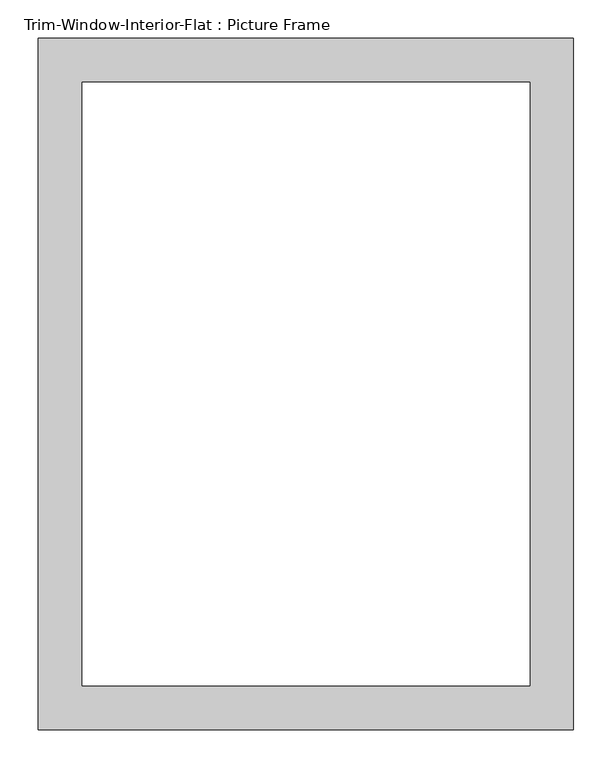
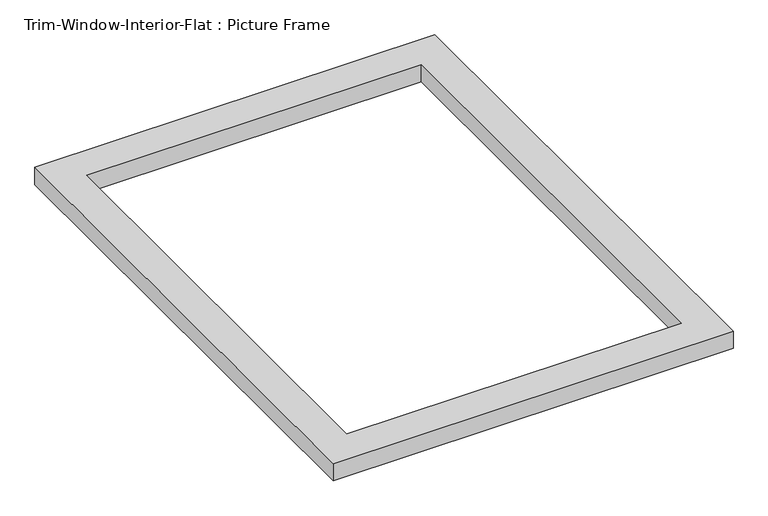
"""IFC4 building model written with IfcOpenShell, lengths in millimetres: proxy geometry, Trim-Window-Interior-Flat : Picture Frame."""

import ifcopenshell
import ifcopenshell.guid

model = None  # the IFC model being written
_history = None  # IfcOwnerHistory: only IFC2X3 demands one
_inside = {}  # id of a spatial element -> (the spatial element, [elements in it])
_under = {}  # id of a project, library or spatial element -> (it, [spatial elements below it])
_declared = {}  # id of a project -> (the project, [libraries it declares])
_typed = {}  # id of a type object -> (the type object, [elements of that type])
_made_of = {}  # id of a material, layer set ... -> (it, [elements and type objects made of it])


def new_model(schema):
    """Start an empty IFC model of exactly this schema.

    Asked for "IFC4X3", IfcOpenShell would pick the latest addendum, in which some entities
    have other attributes; the version numbers below select the first issue.
    IFC2X3 requires an IfcOwnerHistory on every rooted entity: one is made here for all.
    """
    global model, _history
    if schema == "IFC4X3":
        model = ifcopenshell.file(schema_version=(4, 3, 0, 0))
    else:
        model = ifcopenshell.file(schema=schema)
    _inside.clear()
    _under.clear()
    _declared.clear()
    _typed.clear()
    _made_of.clear()
    _history = None
    if model.schema == "IFC2X3":
        org = make("IfcOrganization", Name="unknown")
        user = make(
            "IfcPersonAndOrganization",
            ThePerson=make("IfcPerson", FamilyName="unknown"),
            TheOrganization=org,
        )
        app = make(
            "IfcApplication",
            ApplicationDeveloper=org,
            Version="unknown",
            ApplicationFullName="unknown",
            ApplicationIdentifier="unknown",
        )
        _history = make(
            "IfcOwnerHistory",
            OwningUser=user,
            OwningApplication=app,
            ChangeAction="ADDED",
            CreationDate=0,
        )
    return model


def make(cls, **values):
    """One entity of the class cls with the attributes given. An attribute that is None is left unset."""
    return model.create_entity(
        cls, **{name: value for name, value in values.items() if value is not None}
    )


def rooted(cls, **values):
    """An entity with a GlobalId (a new one), such as an element, a storey or a relation."""
    return make(cls, GlobalId=ifcopenshell.guid.new(), OwnerHistory=_history, **values)


def si_unit(unit_type, name, prefix=None):
    """IfcSIUnit, for example si_unit("LENGTHUNIT", "METRE", prefix="MILLI")."""
    return make("IfcSIUnit", UnitType=unit_type, Prefix=prefix, Name=name)


def assignment(units):
    """IfcUnitAssignment: the units of a project."""
    return None if units is None else make("IfcUnitAssignment", Units=units)


def point(xyz):
    """IfcCartesianPoint."""
    return None if xyz is None else make("IfcCartesianPoint", Coordinates=xyz)


def direction(xyz):
    """IfcDirection."""
    return None if xyz is None else make("IfcDirection", DirectionRatios=xyz)


def frame(location, z_axis=None, x_axis=None):
    """IfcAxis2Placement3D, a coordinate frame: its origin and axes. An axis left out is left unset."""
    return make(
        "IfcAxis2Placement3D",
        Location=point(location),
        Axis=direction(z_axis),
        RefDirection=direction(x_axis),
    )


def origin():
    """The frame at (0, 0, 0) with its axes left unset."""
    return frame((0.0, 0.0, 0.0))


def origin_with_axes():
    """The frame at (0, 0, 0) with the z axis (0, 0, 1) and the x axis (1, 0, 0) written out."""
    return frame((0.0, 0.0, 0.0), z_axis=(0.0, 0.0, 1.0), x_axis=(1.0, 0.0, 0.0))


def place(relative_to, where):
    """IfcLocalPlacement: puts the frame where relative to a parent placement (None: the world)."""
    return make(
        "IfcLocalPlacement", PlacementRelTo=relative_to, RelativePlacement=where
    )


def context(
    kind, dimensions, precision=None, world=None, true_north=None, identifier=None
):
    """IfcGeometricRepresentationContext, for example the 3D "Model" context."""
    return make(
        "IfcGeometricRepresentationContext",
        ContextIdentifier=identifier,
        ContextType=kind,
        CoordinateSpaceDimension=dimensions,
        Precision=precision,
        WorldCoordinateSystem=world,
        TrueNorth=true_north,
    )


def project(units=None, contexts=None):
    """IfcProject with its units and contexts."""
    return rooted(
        "IfcProject",
        Name="project",
        RepresentationContexts=contexts,
        UnitsInContext=assignment(units),
    )


def spatial(cls, under=None, at=None, **own):
    """A site, building, storey or space (cls), placed at a placement, below another one or the project."""
    s = rooted(cls, ObjectPlacement=at, **own)
    if under is not None:
        _under.setdefault(under.id(), (under, []))[1].append(s)
    return s


def polyline(points):
    """IfcPolyline through the points."""
    return make("IfcPolyline", Points=[point(p) for p in points])


def outline(outer, holes=None, kind="AREA"):
    """IfcArbitraryClosedProfileDef: a profile drawn as a closed curve; with holes, ...WithVoids."""
    if holes is None:
        return make("IfcArbitraryClosedProfileDef", ProfileType=kind, OuterCurve=outer)
    return make(
        "IfcArbitraryProfileDefWithVoids",
        ProfileType=kind,
        OuterCurve=outer,
        InnerCurves=holes,
    )


def extrude(swept, where, along, depth):
    """IfcExtrudedAreaSolid: the profile swept, set in the frame where, extruded along a direction by depth."""
    return make(
        "IfcExtrudedAreaSolid",
        SweptArea=swept,
        Position=where,
        ExtrudedDirection=direction(along),
        Depth=depth,
    )


def shape(context_of_items, identifier, shape_type, items):
    """IfcShapeRepresentation: the items that make up one representation, for example the "Body"."""
    return make(
        "IfcShapeRepresentation",
        ContextOfItems=context_of_items,
        RepresentationIdentifier=identifier,
        RepresentationType=shape_type,
        Items=items,
    )


def source(mapping_origin, context_of_items, identifier, shape_type, items):
    """IfcRepresentationMap: a shape defined once, which mapped items show again and again."""
    return make(
        "IfcRepresentationMap",
        MappingOrigin=mapping_origin,
        MappedRepresentation=shape(context_of_items, identifier, shape_type, items),
    )


def transform(
    local_origin,
    x_axis=None,
    y_axis=None,
    z_axis=None,
    scale=None,
    scale2=None,
    scale3=None,
    uniform=True,
):
    """IfcCartesianTransformationOperator3D, or its non-uniform kind. x_axis, y_axis, z_axis: its Axis1, 2, 3."""
    if uniform:
        return make(
            "IfcCartesianTransformationOperator3D",
            Axis1=direction(x_axis),
            Axis2=direction(y_axis),
            LocalOrigin=point(local_origin),
            Scale=scale,
            Axis3=direction(z_axis),
        )
    return make(
        "IfcCartesianTransformationOperator3DnonUniform",
        Axis1=direction(x_axis),
        Axis2=direction(y_axis),
        LocalOrigin=point(local_origin),
        Scale=scale,
        Axis3=direction(z_axis),
        Scale2=scale2,
        Scale3=scale3,
    )


def mapped(mapping_source, mapping_target):
    """IfcMappedItem: shows the shape of a source again, moved by a transform."""
    return make(
        "IfcMappedItem", MappingSource=mapping_source, MappingTarget=mapping_target
    )


def made_of(thing, what):
    """Note that an element or type object is made of a material, layer set ...; save() writes the relation."""
    if what is not None:
        _made_of.setdefault(what.id(), (what, []))[1].append(thing)
    return thing


def element(
    cls,
    number,
    at=None,
    inside=None,
    cuts=None,
    type_object=None,
    material=None,
    context=None,
    identifier="Body",
    shape_type=None,
    held_by="IfcProductDefinitionShape",
    body=None,
    shapes=None,
    **own,
):
    """One element of the class cls, such as IfcWall. Its Tag is "e" and its number.

    at: its placement. inside: the storey or other place that contains it. cuts: it is an
    opening in that element (IfcRelVoidsElement). A single representation is given by context,
    identifier, shape_type and body (its items); several are given by shapes. held_by: the class
    of the entity that holds the representations. save() writes the other relations.
    """
    e = rooted(cls, Tag="e%d" % number, ObjectPlacement=at, **own)
    if body is not None:
        shapes = [shape(context, identifier, shape_type, body)]
    if shapes is not None:
        e.Representation = make(held_by, Representations=shapes)
    if inside is not None:
        _inside.setdefault(inside.id(), (inside, []))[1].append(e)
    if cuts is not None:
        rooted(
            "IfcRelVoidsElement", RelatingBuildingElement=cuts, RelatedOpeningElement=e
        )
    if type_object is not None:
        _typed.setdefault(type_object.id(), (type_object, []))[1].append(e)
    return made_of(e, material)


def aggregate(whole, parts):
    """IfcRelAggregates: a whole, such as a stair, and the parts it consists of."""
    return rooted("IfcRelAggregates", RelatingObject=whole, RelatedObjects=parts)


def save(model, path):
    """Write the relations noted so far, then the file.

    IfcRelAggregates (storeys below a building ...), IfcRelContainedInSpatialStructure (elements
    in a storey), IfcRelDefinesByType, IfcRelAssociatesMaterial and IfcRelDeclares: one each for
    every whole, place, type object, material and project.
    """
    for whole, parts in _under.values():
        aggregate(whole, parts)
    for where, things in _inside.values():
        rooted(
            "IfcRelContainedInSpatialStructure",
            RelatedElements=things,
            RelatingStructure=where,
        )
    for kind, things in _typed.values():
        rooted("IfcRelDefinesByType", RelatedObjects=things, RelatingType=kind)
    for what, things in _made_of.values():
        rooted("IfcRelAssociatesMaterial", RelatedObjects=things, RelatingMaterial=what)
    for by, libraries in _declared.values():
        rooted("IfcRelDeclares", RelatingContext=by, RelatedDefinitions=libraries)
    model.write(path)


def trim_window_interior_flat_picture_frame_6a74a1f9(model_context):
    return source(origin(), model_context, "Body", "SweptSolid", [
        extrude(outline(polyline([(349.25, 44.45), (349.25, -857.25), (-349.25, -857.25), (-349.25, 44.45), (349.25, 44.45)]), holes=[polyline([(292.1, -12.7), (-292.1, -12.7), (-292.1, -800.1), (292.1, -800.1), (292.1, -12.7)])]), origin_with_axes(), (0.0, 0.0, 1.0), 31.75),
    ])


if __name__ == "__main__":
    model = new_model("IFC4")
    model_context = context("Model", 3, world=origin())
    ifc_project = project(units=[si_unit("LENGTHUNIT", "METRE", prefix="MILLI")], contexts=[model_context])
    site = spatial("IfcSite", under=ifc_project)
    building = spatial("IfcBuilding", under=site)
    placement = place(None, origin())
    trim_window_interior_flat_picture_frame_shape = trim_window_interior_flat_picture_frame_6a74a1f9(model_context)
    element("IfcBuildingElementProxy", 1, Name="Trim-Window-Interior-Flat : Picture Frame", ObjectType="Trim-Window-Interior-Flat : Picture Frame", at=placement, inside=building, context=model_context, shape_type="MappedRepresentation", body=[
        mapped(trim_window_interior_flat_picture_frame_shape, transform((0.0, 0.0, 0.0), x_axis=(1.0, 0.0, 0.0), y_axis=(0.0, 1.0, 0.0), z_axis=(0.0, 0.0, 1.0))),
    ])
    save(model, "model.ifc")

# Revit data of these elements
# Type "Trim-Window-Interior-Flat : Picture Frame"
#   Trim Thickness_Picture Frame = 0' - 1 1/4"
#   Trim Width = 0' - 2 1/4"
#   Trim Thickness_with Sill = 0' - 0 3/4"
#   Sill Thickness = 0' - 1 1/4"
#   Opening Width [instance default] = 2' - 0"
#   Opening Height [instance default] = 3' - 0"
#   Default Elevation = 4' - 0"
#   Sill = no
#   Picture Frame = yes
#   Trim Material [instance default] = none
# Element 1 (IfcBuildingElementProxy, "Trim-Window-Interior-Flat : Picture Frame")
#   Opening Height = 2' - 8"
#   Trim Material = Wood - Stained
#   Materials on its faces: "Wood - Stained"
# Materials
#   "Wood - Stained": class "Wood", colour RGB 224 178 126, transparency 0, Cost = 0
